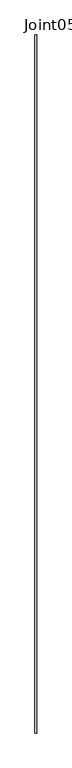
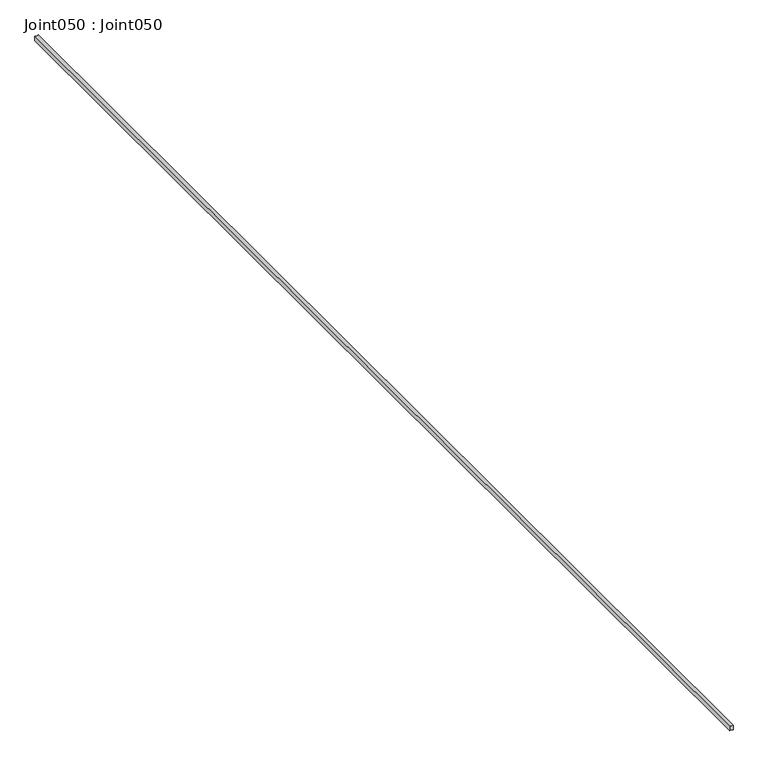
"""IFC4 building model written with IfcOpenShell, lengths in millimetres: proxy geometry, Joint050 : Joint050."""

from ifc_helpers import new_model, si_unit, point, frame, frame_2d, origin, place, context, project, spatial, polyline, circle_curve, trimmed, segment, composite_curve, outline, extrude, source, transform, mapped, element, save


def joint050_joint050_c4e0bbcc(model_context):
    return source(origin(), model_context, "Body", "SweptSolid", [
        extrude(outline(composite_curve([segment(polyline([(43736.5432875, 6057.1640491), (43744.6425585, 6057.1638412)]), True, "CONTINUOUS"), segment(trimmed(circle_curve(frame_2d((43747.6529615, 6054.2179852)), 4.2119584), [point((43744.6425585, 6057.1638412))], [point((43744.6425585, 6051.2721293))], True, "CARTESIAN"), True, "CONTINUOUS"), segment(polyline([(43744.6425585, 6051.2721293), (43736.5432875, 6051.2721293)]), True, "CONTINUOUS"), segment(trimmed(circle_curve(frame_2d((43729.3954638, 6054.2180892)), 7.7311101), [point((43736.5432875, 6051.2721293))], [point((43736.5432875, 6057.1640491))], True, "CARTESIAN"), True, "CONTINUOUS")], self_intersect=False)), frame((0.0, -1052.891, 0.0), z_axis=(0.0, 1.0, 0.0), x_axis=(0.0, 0.0, 1.0)), (0.0, 0.0, 1.0), 2000.0),
    ])


if __name__ == "__main__":
    model = new_model("IFC4")
    model_context = context("Model", 3, world=origin())
    ifc_project = project(units=[si_unit("LENGTHUNIT", "METRE", prefix="MILLI")], contexts=[model_context])
    site = spatial("IfcSite", under=ifc_project)
    building = spatial("IfcBuilding", under=site)
    placement = place(None, origin())
    joint050_joint050_shape = joint050_joint050_c4e0bbcc(model_context)
    element("IfcBuildingElementProxy", 1, Name="Joint050 : Joint050", ObjectType="Joint050 : Joint050", at=placement, inside=building, context=model_context, shape_type="MappedRepresentation", body=[
        mapped(joint050_joint050_shape, transform((0.0, 0.0, 0.0), x_axis=(1.0, 0.0, 0.0), y_axis=(0.0, 1.0, 0.0), z_axis=(0.0, 0.0, 1.0))),
    ])
    save(model, "model.ifc")

# Revit data of these elements
# Type "Joint050 : Joint050"
#   NameOverride = "Joint050"
# Element 1 (IfcBuildingElementProxy, "Joint050 : Joint050")
#   Materials on its faces: "SEALANT"
# Materials
#   "SEALANT": class "Unassigned", colour RGB 142 225 148, transparency 0
